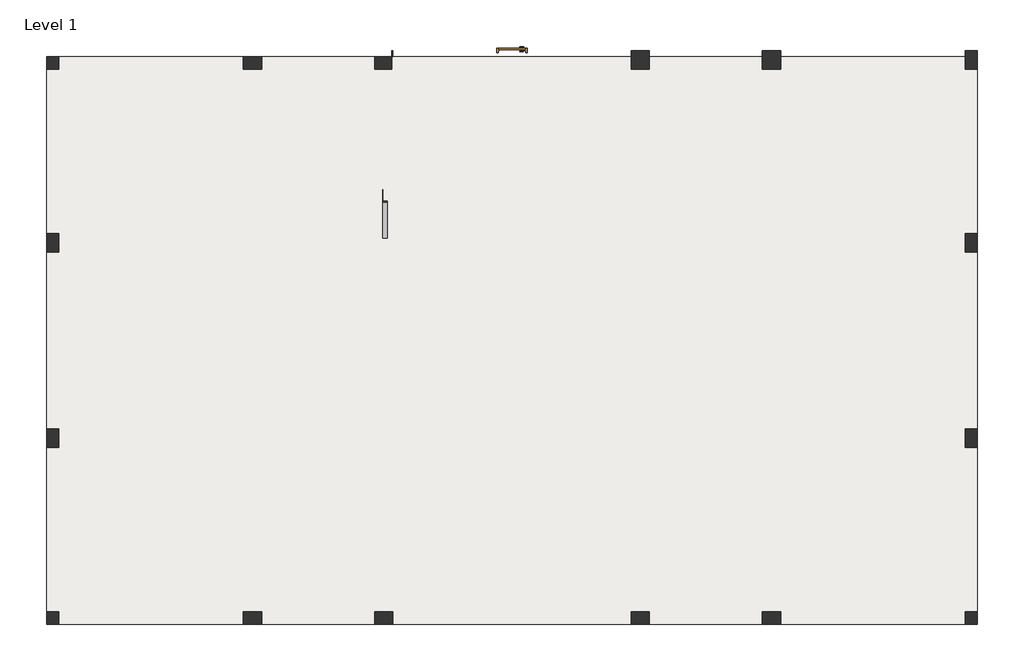
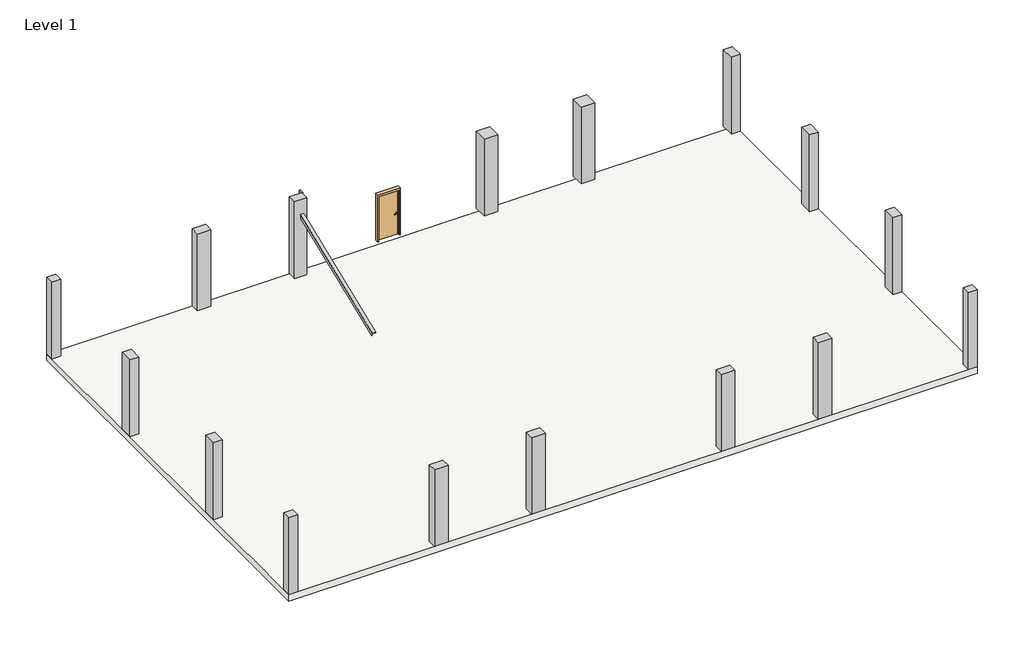
# One storey: 16 columns, 1 door, 1 member, 1 slab.
"""IFC4 building model written with IfcOpenShell, lengths in millimetres."""

import ifcopenshell
import ifcopenshell.guid

model = None  # the IFC model being written
_history = None  # IfcOwnerHistory: only IFC2X3 demands one
_inside = {}  # id of a spatial element -> (the spatial element, [elements in it])
_under = {}  # id of a project, library or spatial element -> (it, [spatial elements below it])
_declared = {}  # id of a project -> (the project, [libraries it declares])
_typed = {}  # id of a type object -> (the type object, [elements of that type])
_made_of = {}  # id of a material, layer set ... -> (it, [elements and type objects made of it])


def new_model(schema):
    """Start an empty IFC model of exactly this schema.

    Asked for "IFC4X3", IfcOpenShell would pick the latest addendum, in which some entities
    have other attributes; the version numbers below select the first issue.
    IFC2X3 requires an IfcOwnerHistory on every rooted entity: one is made here for all.
    """
    global model, _history
    if schema == "IFC4X3":
        model = ifcopenshell.file(schema_version=(4, 3, 0, 0))
    else:
        model = ifcopenshell.file(schema=schema)
    _inside.clear()
    _under.clear()
    _declared.clear()
    _typed.clear()
    _made_of.clear()
    _history = None
    if model.schema == "IFC2X3":
        org = make("IfcOrganization", Name="unknown")
        user = make(
            "IfcPersonAndOrganization",
            ThePerson=make("IfcPerson", FamilyName="unknown"),
            TheOrganization=org,
        )
        app = make(
            "IfcApplication",
            ApplicationDeveloper=org,
            Version="unknown",
            ApplicationFullName="unknown",
            ApplicationIdentifier="unknown",
        )
        _history = make(
            "IfcOwnerHistory",
            OwningUser=user,
            OwningApplication=app,
            ChangeAction="ADDED",
            CreationDate=0,
        )
    return model


def make(cls, **values):
    """One entity of the class cls with the attributes given. An attribute that is None is left unset."""
    return model.create_entity(
        cls, **{name: value for name, value in values.items() if value is not None}
    )


def rooted(cls, **values):
    """An entity with a GlobalId (a new one), such as an element, a storey or a relation."""
    return make(cls, GlobalId=ifcopenshell.guid.new(), OwnerHistory=_history, **values)


def si_unit(unit_type, name, prefix=None):
    """IfcSIUnit, for example si_unit("LENGTHUNIT", "METRE", prefix="MILLI")."""
    return make("IfcSIUnit", UnitType=unit_type, Prefix=prefix, Name=name)


def assignment(units):
    """IfcUnitAssignment: the units of a project."""
    return None if units is None else make("IfcUnitAssignment", Units=units)


def point(xyz):
    """IfcCartesianPoint."""
    return None if xyz is None else make("IfcCartesianPoint", Coordinates=xyz)


def direction(xyz):
    """IfcDirection."""
    return None if xyz is None else make("IfcDirection", DirectionRatios=xyz)


def frame(location, z_axis=None, x_axis=None):
    """IfcAxis2Placement3D, a coordinate frame: its origin and axes. An axis left out is left unset."""
    return make(
        "IfcAxis2Placement3D",
        Location=point(location),
        Axis=direction(z_axis),
        RefDirection=direction(x_axis),
    )


def frame_2d(location, x_axis=None):
    """IfcAxis2Placement2D, a coordinate frame in the plane: its origin and x axis."""
    return make(
        "IfcAxis2Placement2D", Location=point(location), RefDirection=direction(x_axis)
    )


def origin():
    """The frame at (0, 0, 0) with its axes left unset."""
    return frame((0.0, 0.0, 0.0))


def origin_with_axes():
    """The frame at (0, 0, 0) with the z axis (0, 0, 1) and the x axis (1, 0, 0) written out."""
    return frame((0.0, 0.0, 0.0), z_axis=(0.0, 0.0, 1.0), x_axis=(1.0, 0.0, 0.0))


def place(relative_to, where):
    """IfcLocalPlacement: puts the frame where relative to a parent placement (None: the world)."""
    return make(
        "IfcLocalPlacement", PlacementRelTo=relative_to, RelativePlacement=where
    )


def context(
    kind, dimensions, precision=None, world=None, true_north=None, identifier=None
):
    """IfcGeometricRepresentationContext, for example the 3D "Model" context."""
    return make(
        "IfcGeometricRepresentationContext",
        ContextIdentifier=identifier,
        ContextType=kind,
        CoordinateSpaceDimension=dimensions,
        Precision=precision,
        WorldCoordinateSystem=world,
        TrueNorth=true_north,
    )


def project(units=None, contexts=None):
    """IfcProject with its units and contexts."""
    return rooted(
        "IfcProject",
        Name="project",
        RepresentationContexts=contexts,
        UnitsInContext=assignment(units),
    )


def spatial(cls, under=None, at=None, **own):
    """A site, building, storey or space (cls), placed at a placement, below another one or the project."""
    s = rooted(cls, ObjectPlacement=at, **own)
    if under is not None:
        _under.setdefault(under.id(), (under, []))[1].append(s)
    return s


def polyline(points):
    """IfcPolyline through the points."""
    return make("IfcPolyline", Points=[point(p) for p in points])


def circle_curve(where, radius):
    """IfcCircle in the frame where."""
    return make("IfcCircle", Position=where, Radius=radius)


def ellipse_curve(where, semi_axis1, semi_axis2):
    """IfcEllipse in the frame where."""
    return make(
        "IfcEllipse", Position=where, SemiAxis1=semi_axis1, SemiAxis2=semi_axis2
    )


def trimmed(basis, trim1, trim2, sense, master):
    """IfcTrimmedCurve: the piece of a basis curve between two trims."""
    return make(
        "IfcTrimmedCurve",
        BasisCurve=basis,
        Trim1=trim1,
        Trim2=trim2,
        SenseAgreement=sense,
        MasterRepresentation=master,
    )


def segment(curve, same_sense, transition):
    """IfcCompositeCurveSegment."""
    return make(
        "IfcCompositeCurveSegment",
        Transition=transition,
        SameSense=same_sense,
        ParentCurve=curve,
    )


def composite_curve(segments, self_intersect=None):
    """IfcCompositeCurve: segments joined end to end."""
    return make("IfcCompositeCurve", Segments=segments, SelfIntersect=self_intersect)


def outline(outer, holes=None, kind="AREA"):
    """IfcArbitraryClosedProfileDef: a profile drawn as a closed curve; with holes, ...WithVoids."""
    if holes is None:
        return make("IfcArbitraryClosedProfileDef", ProfileType=kind, OuterCurve=outer)
    return make(
        "IfcArbitraryProfileDefWithVoids",
        ProfileType=kind,
        OuterCurve=outer,
        InnerCurves=holes,
    )


def extrude(swept, where, along, depth):
    """IfcExtrudedAreaSolid: the profile swept, set in the frame where, extruded along a direction by depth."""
    return make(
        "IfcExtrudedAreaSolid",
        SweptArea=swept,
        Position=where,
        ExtrudedDirection=direction(along),
        Depth=depth,
    )


def faces_of(points, faces, orient=None, outer=None):
    """IfcFace entities. A face is a list of loops; a loop is a list of indices into points, from 0.

    orient and outer hold one flag for each loop. By default every Orientation is true, the
    first loop of a face is its IfcFaceOuterBound and the others are IfcFaceBound.
    """
    made = []
    for i, loops in enumerate(faces):
        bounds = []
        for j, loop in enumerate(loops):
            is_outer = j == 0 if outer is None else outer[i][j]
            bounds.append(
                make(
                    "IfcFaceOuterBound" if is_outer else "IfcFaceBound",
                    Bound=make("IfcPolyLoop", Polygon=[points[k] for k in loop]),
                    Orientation=True if orient is None else orient[i][j],
                )
            )
        made.append(make("IfcFace", Bounds=bounds))
    return made


def faceted_brep(points, faces, orient=None, outer=None, voids=None):
    """IfcFacetedBrep: a solid bounded by flat faces; with voids (closed shells), ...WithVoids."""
    shared = [point(p) for p in points]
    hull = make("IfcClosedShell", CfsFaces=faces_of(shared, faces, orient, outer))
    if voids is None:
        return make("IfcFacetedBrep", Outer=hull)
    return make(
        "IfcFacetedBrepWithVoids",
        Outer=hull,
        Voids=[
            make(cls, CfsFaces=faces_of(shared, fs, o, b)) for cls, fs, o, b in voids
        ],
    )


def shape(context_of_items, identifier, shape_type, items):
    """IfcShapeRepresentation: the items that make up one representation, for example the "Body"."""
    return make(
        "IfcShapeRepresentation",
        ContextOfItems=context_of_items,
        RepresentationIdentifier=identifier,
        RepresentationType=shape_type,
        Items=items,
    )


def source(mapping_origin, context_of_items, identifier, shape_type, items):
    """IfcRepresentationMap: a shape defined once, which mapped items show again and again."""
    return make(
        "IfcRepresentationMap",
        MappingOrigin=mapping_origin,
        MappedRepresentation=shape(context_of_items, identifier, shape_type, items),
    )


def transform(
    local_origin,
    x_axis=None,
    y_axis=None,
    z_axis=None,
    scale=None,
    scale2=None,
    scale3=None,
    uniform=True,
):
    """IfcCartesianTransformationOperator3D, or its non-uniform kind. x_axis, y_axis, z_axis: its Axis1, 2, 3."""
    if uniform:
        return make(
            "IfcCartesianTransformationOperator3D",
            Axis1=direction(x_axis),
            Axis2=direction(y_axis),
            LocalOrigin=point(local_origin),
            Scale=scale,
            Axis3=direction(z_axis),
        )
    return make(
        "IfcCartesianTransformationOperator3DnonUniform",
        Axis1=direction(x_axis),
        Axis2=direction(y_axis),
        LocalOrigin=point(local_origin),
        Scale=scale,
        Axis3=direction(z_axis),
        Scale2=scale2,
        Scale3=scale3,
    )


def mapped(mapping_source, mapping_target):
    """IfcMappedItem: shows the shape of a source again, moved by a transform."""
    return make(
        "IfcMappedItem", MappingSource=mapping_source, MappingTarget=mapping_target
    )


def made_of(thing, what):
    """Note that an element or type object is made of a material, layer set ...; save() writes the relation."""
    if what is not None:
        _made_of.setdefault(what.id(), (what, []))[1].append(thing)
    return thing


def element(
    cls,
    number,
    at=None,
    inside=None,
    cuts=None,
    type_object=None,
    material=None,
    context=None,
    identifier="Body",
    shape_type=None,
    held_by="IfcProductDefinitionShape",
    body=None,
    shapes=None,
    **own,
):
    """One element of the class cls, such as IfcWall. Its Tag is "e" and its number.

    at: its placement. inside: the storey or other place that contains it. cuts: it is an
    opening in that element (IfcRelVoidsElement). A single representation is given by context,
    identifier, shape_type and body (its items); several are given by shapes. held_by: the class
    of the entity that holds the representations. save() writes the other relations.
    """
    e = rooted(cls, Tag="e%d" % number, ObjectPlacement=at, **own)
    if body is not None:
        shapes = [shape(context, identifier, shape_type, body)]
    if shapes is not None:
        e.Representation = make(held_by, Representations=shapes)
    if inside is not None:
        _inside.setdefault(inside.id(), (inside, []))[1].append(e)
    if cuts is not None:
        rooted(
            "IfcRelVoidsElement", RelatingBuildingElement=cuts, RelatedOpeningElement=e
        )
    if type_object is not None:
        _typed.setdefault(type_object.id(), (type_object, []))[1].append(e)
    return made_of(e, material)


def aggregate(whole, parts):
    """IfcRelAggregates: a whole, such as a stair, and the parts it consists of."""
    return rooted("IfcRelAggregates", RelatingObject=whole, RelatedObjects=parts)


def save(model, path):
    """Write the relations noted so far, then the file.

    IfcRelAggregates (storeys below a building ...), IfcRelContainedInSpatialStructure (elements
    in a storey), IfcRelDefinesByType, IfcRelAssociatesMaterial and IfcRelDeclares: one each for
    every whole, place, type object, material and project.
    """
    for whole, parts in _under.values():
        aggregate(whole, parts)
    for where, things in _inside.values():
        rooted(
            "IfcRelContainedInSpatialStructure",
            RelatedElements=things,
            RelatingStructure=where,
        )
    for kind, things in _typed.values():
        rooted("IfcRelDefinesByType", RelatedObjects=things, RelatingType=kind)
    for what, things in _made_of.values():
        rooted("IfcRelAssociatesMaterial", RelatedObjects=things, RelatingMaterial=what)
    for by, libraries in _declared.values():
        rooted("IfcRelDeclares", RelatingContext=by, RelatedDefinitions=libraries)
    model.write(path)


def plane_surface(at):
    """IfcPlane: the flat surface through the origin of the frame at, square to its z axis."""
    return make("IfcPlane", Position=at)


def cylinder_surface(at, radius):
    """IfcCylindricalSurface: all points at the distance radius from the z axis of the frame at."""
    return make("IfcCylindricalSurface", Position=at, Radius=radius)


def revolved_surface(curve, axis_point, axis_direction):
    """IfcSurfaceOfRevolution: the curve turned about the line through axis_point along axis_direction."""
    return make(
        "IfcSurfaceOfRevolution",
        SweptCurve=make("IfcArbitraryOpenProfileDef", ProfileType="CURVE", Curve=curve),
        AxisPosition=make("IfcAxis1Placement", Location=point(axis_point), Axis=direction(axis_direction)),
    )


def advanced_brep(points, edges, surfaces, faces):
    """IfcAdvancedBrep: a solid bounded by faces that lie on surfaces and meet in shared edges.

    An edge is (start, end): straight between two places in points (the first is 0);
    or (start, end, curve); or (start, end, curve, False) where it runs against its curve.
    A face is (place in surfaces, loops), or (place, loops, False) where it looks against
    its surface's normal. A loop lists edges by number (the first is 1), with a minus sign
    where the edge is run from its end to its start. The first loop is the outer one.
    """
    corners = [point(p) for p in points]
    vertices = [make("IfcVertexPoint", VertexGeometry=c) for c in corners]
    made = []
    for start, end, *more in edges:
        made.append(
            make(
                "IfcEdgeCurve",
                EdgeStart=vertices[start],
                EdgeEnd=vertices[end],
                EdgeGeometry=more[0] if more else make("IfcPolyline", Points=[corners[start], corners[end]]),
                SameSense=more[1] if len(more) > 1 else True,
            )
        )
    hull = []
    for where, loops, *sense in faces:
        bounds = []
        for j, loop in enumerate(loops):
            ring = [make("IfcOrientedEdge", EdgeElement=made[abs(k) - 1], Orientation=k > 0) for k in loop]
            bounds.append(
                make(
                    "IfcFaceOuterBound" if j == 0 else "IfcFaceBound",
                    Bound=make("IfcEdgeLoop", EdgeList=ring),
                    Orientation=True,
                )
            )
        hull.append(make("IfcAdvancedFace", Bounds=bounds, FaceSurface=surfaces[where], SameSense=sense[0] if sense else True))
    return make("IfcAdvancedBrep", Outer=make("IfcClosedShell", CfsFaces=hull))


def door_58febf71(model_context):
    return source(origin(), model_context, "Body", "SolidModel", [
        advanced_brep(
        [(-392.190625, -76.1375, 1016.0), (-372.190625, -76.1375, 1016.0), (-392.190625, -46.1375, 1016.0), (-372.190625, -46.1375, 1016.0), (-367.190625, -41.1375, 1016.0), (-367.190625, -21.1375, 1016.0), (-262.190625, -21.1375, 1016.0), (-262.190625, -41.1375, 1016.0)],
        [
            (0, 1, circle_curve(frame((-382.190625, -76.1375, 1016.0), z_axis=(0.0, -1.0, 0.0), x_axis=(1.0, 0.0, 0.0)), 10.0)),
            (1, 0, circle_curve(frame((-382.190625, -76.1375, 1016.0), z_axis=(0.0, -1.0, 0.0), x_axis=(1.0, 0.0, 0.0)), 10.0)),
            (0, 2),
            (2, 3, circle_curve(frame((-382.190625, -46.1375, 1016.0), z_axis=(0.0, -1.0, 0.0), x_axis=(1.0, 0.0, 0.0)), 10.0)),
            (3, 1),
            (3, 2, circle_curve(frame((-382.190625, -46.1375, 1016.0), z_axis=(0.0, -1.0, 0.0), x_axis=(1.0, 0.0, 0.0)), 10.0)),
            (4, 3, circle_curve(frame((-367.190625, -46.1375, 1016.0), z_axis=(0.0, 0.0, 1.0), x_axis=(-1.0, 0.0, 0.0)), 5.0)),
            (2, 5, circle_curve(frame((-367.190625, -46.1375, 1016.0), z_axis=(0.0, 0.0, -1.0), x_axis=(-1.0, 0.0, 0.0)), 25.0)),
            (5, 4, circle_curve(frame((-367.190625, -31.1375, 1016.0), z_axis=(-1.0, 0.0, 0.0), x_axis=(0.0, -1.0, 0.0)), 10.0)),
            (4, 5, circle_curve(frame((-367.190625, -31.1375, 1016.0), z_axis=(-1.0, 0.0, 0.0), x_axis=(0.0, -1.0, 0.0)), 10.0)),
            (6, 7, circle_curve(frame((-262.190625, -31.1375, 1016.0), z_axis=(1.0, 0.0, 0.0), x_axis=(0.0, -1.0, 0.0)), 10.0)),
            (7, 6, circle_curve(frame((-262.190625, -31.1375, 1016.0), z_axis=(1.0, 0.0, 0.0), x_axis=(0.0, -1.0, 0.0)), 10.0)),
            (5, 6),
            (7, 4),
        ],
        [
            plane_surface(frame((-382.190625, -76.1375, 1016.0), z_axis=(0.0, -1.0, 0.0), x_axis=(0.0, 0.0, 1.0))),
            cylinder_surface(frame((-382.190625, -76.1375, 1016.0), z_axis=(0.0, -1.0, 0.0), x_axis=(1.0, 0.0, 0.0)), 10.0),
            revolved_surface(trimmed(ellipse_curve(frame((-382.190625, -46.1375, 1016.0), z_axis=(0.0, -1.0, 0.0), x_axis=(1.0, 0.0, 0.0)), 10.0, 10.0), [point((-392.190625, -46.1375, 1016.0))], [point((-372.190625, -46.1375, 1016.0))], True, "CARTESIAN"), (-367.190625, -46.1375, 1016.0), (0.0, 0.0, -1.0)),
            revolved_surface(trimmed(ellipse_curve(frame((-382.190625, -46.1375, 1016.0), z_axis=(0.0, -1.0, 0.0), x_axis=(1.0, 0.0, 0.0)), 10.0, 10.0), [point((-372.190625, -46.1375, 1016.0))], [point((-392.190625, -46.1375, 1016.0))], True, "CARTESIAN"), (-367.190625, -46.1375, 1016.0), (0.0, 0.0, -1.0)),
            plane_surface(frame((-262.190625, -31.1375, 1016.0), z_axis=(1.0, 0.0, 0.0), x_axis=(0.0, 0.0, 1.0))),
            cylinder_surface(frame((-367.190625, -31.1375, 1016.0), z_axis=(-1.0, 0.0, 0.0), x_axis=(0.0, -1.0, 0.0)), 10.0),
        ],
        [
            (0, [[1, 2]]),
            (1, [[-1, 3, 4, 5]]),
            (1, [[-2, -5, 6, -3]]),
            (2, [[7, -4, 8, 9]]),
            (3, [[-8, -6, -7, 10]]),
            (4, [[11, 12]]),
            (5, [[-9, 13, -12, 14]]),
            (5, [[-10, -14, -11, -13]]),
        ],
    ),
        extrude(outline(composite_curve([segment(trimmed(circle_curve(frame_2d((1016.0, -384.690625)), 30.0), [point((1016.0, -414.690625))], [point((1016.0, -354.690625))], False, "CARTESIAN"), True, "CONTINUOUS"), segment(trimmed(circle_curve(frame_2d((1016.0, -384.690625)), 30.0), [point((1016.0, -354.690625))], [point((1016.0, -414.690625))], False, "CARTESIAN"), True, "CONTINUOUS")], self_intersect=False)), frame((0.0, -84.1375, 0.0), z_axis=(0.0, 1.0, 0.0), x_axis=(0.0, 0.0, 1.0)), (0.0, 0.0, 1.0), 8.0),
        advanced_brep(
        [(-392.190625, -136.5875, 1016.0), (-372.190625, -136.5875, 1016.0), (-372.190625, -166.5875, 1016.0), (-392.190625, -166.5875, 1016.0), (-367.190625, -171.5875, 1016.0), (-367.190625, -191.5875, 1016.0), (-262.190625, -191.5875, 1016.0), (-262.190625, -171.5875, 1016.0)],
        [
            (0, 1, circle_curve(frame((-382.190625, -136.5875, 1016.0), z_axis=(0.0, 1.0, 0.0), x_axis=(1.0, 0.0, 0.0)), 10.0)),
            (1, 0, circle_curve(frame((-382.190625, -136.5875, 1016.0), z_axis=(0.0, 1.0, 0.0), x_axis=(1.0, 0.0, 0.0)), 10.0)),
            (1, 2),
            (2, 3, circle_curve(frame((-382.190625, -166.5875, 1016.0), z_axis=(0.0, 1.0, 0.0), x_axis=(1.0, 0.0, 0.0)), 10.0)),
            (3, 0),
            (3, 2, circle_curve(frame((-382.190625, -166.5875, 1016.0), z_axis=(0.0, 1.0, 0.0), x_axis=(1.0, 0.0, 0.0)), 10.0)),
            (4, 5, circle_curve(frame((-367.190625, -181.5875, 1016.0), z_axis=(-1.0, 0.0, 0.0), x_axis=(0.0, 1.0, 0.0)), 10.0)),
            (5, 3, circle_curve(frame((-367.190625, -166.5875, 1016.0), z_axis=(0.0, 0.0, -1.0), x_axis=(-1.0, 0.0, 0.0)), 25.0)),
            (2, 4, circle_curve(frame((-367.190625, -166.5875, 1016.0), z_axis=(0.0, 0.0, 1.0), x_axis=(-1.0, 0.0, 0.0)), 5.0)),
            (5, 4, circle_curve(frame((-367.190625, -181.5875, 1016.0), z_axis=(-1.0, 0.0, 0.0), x_axis=(0.0, 1.0, 0.0)), 10.0)),
            (6, 7, circle_curve(frame((-262.190625, -181.5875, 1016.0), z_axis=(1.0, 0.0, 0.0), x_axis=(0.0, 1.0, 0.0)), 10.0)),
            (7, 6, circle_curve(frame((-262.190625, -181.5875, 1016.0), z_axis=(1.0, 0.0, 0.0), x_axis=(0.0, 1.0, 0.0)), 10.0)),
            (4, 7),
            (6, 5),
        ],
        [
            plane_surface(frame((-382.190625, -136.5875, 1016.0), z_axis=(0.0, 1.0, 0.0), x_axis=(0.0, 0.0, 1.0))),
            cylinder_surface(frame((-382.190625, -136.5875, 1016.0), z_axis=(0.0, 1.0, 0.0), x_axis=(1.0, 0.0, 0.0)), 10.0),
            revolved_surface(trimmed(ellipse_curve(frame((-382.190625, -166.5875, 1016.0), z_axis=(0.0, -1.0, 0.0), x_axis=(1.0, 0.0, 0.0)), 10.0, 10.0), [point((-392.190625, -166.5875, 1016.0))], [point((-372.190625, -166.5875, 1016.0))], True, "CARTESIAN"), (-367.190625, -166.5875, 1016.0), (0.0, 0.0, -1.0)),
            revolved_surface(trimmed(ellipse_curve(frame((-382.190625, -166.5875, 1016.0), z_axis=(0.0, -1.0, 0.0), x_axis=(1.0, 0.0, 0.0)), 10.0, 10.0), [point((-372.190625, -166.5875, 1016.0))], [point((-392.190625, -166.5875, 1016.0))], True, "CARTESIAN"), (-367.190625, -166.5875, 1016.0), (0.0, 0.0, -1.0)),
            plane_surface(frame((-262.190625, -181.5875, 1016.0), z_axis=(1.0, 0.0, 0.0), x_axis=(0.0, 0.0, 1.0))),
            cylinder_surface(frame((-367.190625, -181.5875, 1016.0), z_axis=(-1.0, 0.0, 0.0), x_axis=(0.0, 1.0, 0.0)), 10.0),
        ],
        [
            (0, [[1, 2]]),
            (1, [[3, 4, 5, -2]]),
            (1, [[-5, 6, -3, -1]]),
            (2, [[7, 8, -4, 9]]),
            (3, [[10, -9, -6, -8]]),
            (4, [[11, 12]]),
            (5, [[13, -11, 14, -7]]),
            (5, [[-14, -12, -13, -10]]),
        ],
    ),
        extrude(outline(composite_curve([segment(trimmed(circle_curve(frame_2d((1016.0, -384.690625)), 30.0), [point((1016.0, -414.690625))], [point((1016.0, -354.690625))], False, "CARTESIAN"), True, "CONTINUOUS"), segment(trimmed(circle_curve(frame_2d((1016.0, -384.690625)), 30.0), [point((1016.0, -354.690625))], [point((1016.0, -414.690625))], False, "CARTESIAN"), True, "CONTINUOUS")], self_intersect=False)), frame((0.0, -136.5875, 0.0), z_axis=(0.0, 1.0, 0.0), x_axis=(0.0, 0.0, 1.0)), (0.0, 0.0, 1.0), 8.0),
        faceted_brep([(457.2, -79.375, 0.0), (441.325, -79.375, 0.0), (441.325, -31.75, 0.0), (457.2, -31.75, 0.0), (457.2, 17.4625, 0.0), (508.0, 17.4625, 0.0), (508.0, -128.5875, 0.0), (457.2, -128.5875, 0.0), (457.2, -128.5875, 2133.6), (457.2, -79.375, 2133.6), (508.0, -128.5875, 2235.2), (-508.0, -128.5875, 2235.2), (-508.0, -128.5875, 0.0), (-457.2, -128.5875, 0.0), (-457.2, -128.5875, 2133.6), (508.0, 17.4625, 2235.2), (457.2, 17.4625, 2133.6), (-457.2, 17.4625, 2133.6), (-457.2, 17.4625, 0.0), (-508.0, 17.4625, 0.0), (-508.0, 17.4625, 2235.2), (457.2, -31.75, 2133.6), (441.325, -31.75, 2117.725), (-441.325, -31.75, 2117.725), (-441.325, -31.75, 0.0), (-457.2, -31.75, 0.0), (-457.2, -31.75, 2133.6), (441.325, -79.375, 2117.725), (-457.2, -79.375, 2133.6), (-457.2, -79.375, 0.0), (-441.325, -79.375, 0.0), (-441.325, -79.375, 2117.725)], [[[0, 1, 2, 3, 4, 5, 6, 7]], [[7, 8, 9, 0]], [[6, 10, 11, 12, 13, 14, 8, 7]], [[5, 15, 10, 6]], [[4, 16, 17, 18, 19, 20, 15, 5]], [[3, 21, 16, 4]], [[2, 22, 23, 24, 25, 26, 21, 3]], [[1, 27, 22, 2]], [[0, 9, 28, 29, 30, 31, 27, 1]], [[8, 14, 28, 9]], [[16, 21, 26, 17]], [[22, 27, 31, 23]], [[12, 19, 18, 25, 24, 30, 29, 13]], [[13, 29, 28, 14]], [[11, 20, 19, 12]], [[17, 26, 25, 18]], [[23, 31, 30, 24]], [[15, 20, 11, 10]]]),
        extrude(outline(polyline([(457.2, -84.1375), (457.2, -128.5875), (-457.2, -128.5875), (-457.2, -84.1375), (457.2, -84.1375)])), origin_with_axes(), (0.0, 0.0, 1.0), 2133.6),
    ])


def l_angle_l6x6x3_8_2b984bf3(model_context):
    return source(origin(), model_context, "Body", "SweptSolid", [
        extrude(outline(composite_curve([segment(polyline([(41.148, 41.148), (41.148, -111.252)]), True, "CONTINUOUS"), segment(trimmed(circle_curve(frame_2d((41.148, -101.727)), 9.525), [point((41.148, -111.252))], [point((31.623, -101.727))], False, "CARTESIAN"), True, "CONTINUOUS"), segment(polyline([(31.623, -101.727), (31.623, 22.098)]), True, "CONTINUOUS"), segment(trimmed(circle_curve(frame_2d((22.098, 22.098)), 9.525), [point((31.623, 22.098))], [point((22.098, 31.623))], True, "CARTESIAN"), True, "CONTINUOUS"), segment(polyline([(22.098, 31.623), (-101.727, 31.623)]), True, "CONTINUOUS"), segment(trimmed(circle_curve(frame_2d((-101.727, 41.148)), 9.525), [point((-101.727, 31.623))], [point((-111.252, 41.148))], False, "CARTESIAN"), True, "CONTINUOUS"), segment(polyline([(-111.252, 41.148), (41.148, 41.148)]), True, "CONTINUOUS")], self_intersect=False)), frame((-3088.1296112, 0.0, 0.0), z_axis=(1.0, 0.0, 0.0), x_axis=(0.0, 1.0, 0.0)), (0.0, 0.0, 1.0), 6142.746295),
    ])


model = new_model("IFC4")

# Units and contexts
model_context = context("Model", 3, world=origin())
ifc_project = project(units=[si_unit("LENGTHUNIT", "METRE", prefix="MILLI")], contexts=[model_context])

# Site, building, storey
site = spatial("IfcSite", under=ifc_project)
building = spatial("IfcBuilding", under=site)
storey = spatial("IfcBuildingStorey", under=building, Name="Level 1", Elevation=0.0)

# Columns
placement = place(None, origin())
element("IfcColumn", 1, ObjectType="Rectangular Column : 24\" x 24\"", at=placement, inside=storey, context=model_context, shape_type="SweptSolid", body=[
    extrude(outline(polyline([(-16253.4122732, 9291.5015304), (-16253.4122732, 8885.1015304), (-16659.8122732, 8885.1015304), (-16659.8122732, 9291.5015304), (-16253.4122732, 9291.5015304)])), origin_with_axes(), (0.0, 0.0, 1.0), 3657.6),
])
element("IfcColumn", 2, ObjectType="Rectangular Column : 24\" x 24\"", at=placement, inside=storey, context=model_context, shape_type="SweptSolid", body=[
    extrude(outline(polyline([(-16253.4122732, 3398.7015304), (-16253.4122732, 2789.1015304), (-16659.8122732, 2789.1015304), (-16659.8122732, 3398.7015304), (-16253.4122732, 3398.7015304)])), origin_with_axes(), (0.0, 0.0, 1.0), 3657.6),
])
element("IfcColumn", 3, ObjectType="Rectangular Column : 24\" x 24\"", at=placement, inside=storey, context=model_context, shape_type="SweptSolid", body=[
    extrude(outline(polyline([(-9497.0122732, 8885.1015304), (-10106.6122732, 8885.1015304), (-10106.6122732, 9291.5015304), (-9497.0122732, 9291.5015304), (-9497.0122732, 8885.1015304)])), origin_with_axes(), (0.0, 0.0, 1.0), 3657.6),
])
element("IfcColumn", 4, ObjectType="Rectangular Column : 24\" x 24\"", at=placement, inside=storey, context=model_context, shape_type="SweptSolid", body=[
    extrude(outline(polyline([(-5174.2497732, 9494.7015304), (-5128.2122732, 9494.7015304), (-5128.2122732, 9301.0265304), (-5174.2497732, 9301.0265304), (-5174.2497732, 9494.7015304)])), origin_with_axes(), (0.0, 0.0, 1.0), 3657.6),
    extrude(outline(polyline([(-5737.8122732, 8885.1015304), (-5737.8122732, 9291.5015304), (-5174.2497732, 9291.5015304), (-5174.2497732, 8885.1015304), (-5737.8122732, 8885.1015304)])), origin_with_axes(), (0.0, 0.0, 1.0), 3657.6),
])
element("IfcColumn", 5, ObjectType="Rectangular Column : 24\" x 24\"", at=placement, inside=storey, context=model_context, shape_type="SweptSolid", body=[
    extrude(outline(polyline([(3406.1877268, 9494.7015304), (3406.1877268, 8885.1015304), (2796.5877268, 8885.1015304), (2796.5877268, 9494.7015304), (3406.1877268, 9494.7015304)])), origin_with_axes(), (0.0, 0.0, 1.0), 3657.6),
])
element("IfcColumn", 6, ObjectType="Rectangular Column : 24\" x 24\"", at=placement, inside=storey, context=model_context, shape_type="SweptSolid", body=[
    extrude(outline(polyline([(7774.9877268, 9494.7015304), (7774.9877268, 8885.1015304), (7165.3877268, 8885.1015304), (7165.3877268, 9494.7015304), (7774.9877268, 9494.7015304)])), origin_with_axes(), (0.0, 0.0, 1.0), 3657.6),
])
element("IfcColumn", 7, ObjectType="Rectangular Column : 24\" x 24\"", at=placement, inside=storey, context=model_context, shape_type="SweptSolid", body=[
    extrude(outline(polyline([(13921.7877268, 8885.1015304), (13921.7877268, 9494.7015304), (14328.1877268, 9494.7015304), (14328.1877268, 8885.1015304), (13921.7877268, 8885.1015304)])), origin_with_axes(), (0.0, 0.0, 1.0), 3657.6),
])
element("IfcColumn", 8, ObjectType="Rectangular Column : 24\" x 24\"", at=placement, inside=storey, context=model_context, shape_type="SweptSolid", body=[
    extrude(outline(polyline([(13921.7877268, 2789.1015304), (13921.7877268, 3398.7015304), (14328.1877268, 3398.7015304), (14328.1877268, 2789.1015304), (13921.7877268, 2789.1015304)])), origin_with_axes(), (0.0, 0.0, 1.0), 3657.6),
])
element("IfcColumn", 9, ObjectType="Rectangular Column : 24\" x 24\"", at=placement, inside=storey, context=model_context, shape_type="SweptSolid", body=[
    extrude(outline(polyline([(13921.7877268, -3713.2984696), (13921.7877268, -3103.6984696), (14328.1877268, -3103.6984696), (14328.1877268, -3713.2984696), (13921.7877268, -3713.2984696)])), origin_with_axes(), (0.0, 0.0, 1.0), 3657.6),
])
element("IfcColumn", 10, ObjectType="Rectangular Column : 24\" x 24\"", at=placement, inside=storey, context=model_context, shape_type="SweptSolid", body=[
    extrude(outline(polyline([(13921.7877268, -9606.0984696), (13921.7877268, -9199.6984696), (14328.1877268, -9199.6984696), (14328.1877268, -9606.0984696), (13921.7877268, -9606.0984696)])), origin_with_axes(), (0.0, 0.0, 1.0), 3657.6),
])
element("IfcColumn", 11, ObjectType="Rectangular Column : 24\" x 24\"", at=placement, inside=storey, context=model_context, shape_type="SweptSolid", body=[
    extrude(outline(polyline([(7165.3877268, -9199.6984696), (7774.9877268, -9199.6984696), (7774.9877268, -9606.0984696), (7165.3877268, -9606.0984696), (7165.3877268, -9199.6984696)])), origin_with_axes(), (0.0, 0.0, 1.0), 3657.6),
])
element("IfcColumn", 12, ObjectType="Rectangular Column : 24\" x 24\"", at=placement, inside=storey, context=model_context, shape_type="SweptSolid", body=[
    extrude(outline(polyline([(2796.5877268, -9199.6984696), (3406.1877268, -9199.6984696), (3406.1877268, -9606.0984696), (2796.5877268, -9606.0984696), (2796.5877268, -9199.6984696)])), origin_with_axes(), (0.0, 0.0, 1.0), 3657.6),
])
element("IfcColumn", 13, ObjectType="Rectangular Column : 24\" x 24\"", at=placement, inside=storey, context=model_context, shape_type="SweptSolid", body=[
    extrude(outline(polyline([(-5737.8122732, -9199.6984696), (-5128.2122732, -9199.6984696), (-5128.2122732, -9606.0984696), (-5737.8122732, -9606.0984696), (-5737.8122732, -9199.6984696)])), origin_with_axes(), (0.0, 0.0, 1.0), 3657.6),
])
element("IfcColumn", 14, ObjectType="Rectangular Column : 24\" x 24\"", at=placement, inside=storey, context=model_context, shape_type="SweptSolid", body=[
    extrude(outline(polyline([(-10106.6122732, -9199.6984696), (-9497.0122732, -9199.6984696), (-9497.0122732, -9606.0984696), (-10106.6122732, -9606.0984696), (-10106.6122732, -9199.6984696)])), origin_with_axes(), (0.0, 0.0, 1.0), 3657.6),
])
element("IfcColumn", 15, ObjectType="Rectangular Column : 24\" x 24\"", at=placement, inside=storey, context=model_context, shape_type="SweptSolid", body=[
    extrude(outline(polyline([(-16659.8122732, -9199.6984696), (-16253.4122732, -9199.6984696), (-16253.4122732, -9606.0984696), (-16659.8122732, -9606.0984696), (-16659.8122732, -9199.6984696)])), origin_with_axes(), (0.0, 0.0, 1.0), 3657.6),
])
element("IfcColumn", 16, ObjectType="Rectangular Column : 24\" x 24\"", at=placement, inside=storey, context=model_context, shape_type="SweptSolid", body=[
    extrude(outline(polyline([(-16253.4122732, -3103.6984696), (-16253.4122732, -3713.2984696), (-16659.8122732, -3713.2984696), (-16659.8122732, -3103.6984696), (-16253.4122732, -3103.6984696)])), origin_with_axes(), (0.0, 0.0, 1.0), 3657.6),
])

# Door
door_shape = door_58febf71(model_context)
element("IfcDoor", 17, ObjectType="Door-Passage-Single-Flush : 36\" x 84\"", at=placement, inside=storey, context=model_context, shape_type="MappedRepresentation", body=[
    mapped(door_shape, transform((-1165.8122732, 9442.3140304, 0.0), x_axis=(-1.0, 0.0, 0.0), y_axis=(0.0, -1.0, 0.0), z_axis=(0.0, 0.0, 1.0))),
])

# Member
l_angle_l6x6x3_8_shape = l_angle_l6x6x3_8_2b984bf3(model_context)
element("IfcMember", 18, ObjectType="L-Angle : L6X6X3/8", at=placement, inside=storey, context=model_context, shape_type="MappedRepresentation", body=[
    mapped(l_angle_l6x6x3_8_shape, transform((-5433.0122732, 6141.9015304, 1828.8), x_axis=(0.0, 0.9284766908852565, 0.3713906763541112), y_axis=(-1.0000000000000002, 0.0, 0.0), z_axis=(0.0, -0.3713906763541112, 0.9284766908852565))),
])

# Slab
element("IfcSlab", 19, ObjectType="Generic - 12\"", at=placement, inside=storey, context=model_context, shape_type="SweptSolid", body=[
    extrude(outline(polyline([(-16659.8122732, 9291.5015304), (14328.1877268, 9291.5015304), (14328.1877268, -9606.0984696), (-16659.8122732, -9606.0984696), (-16659.8122732, 9291.5015304)])), frame((0.0, 0.0, -304.8), z_axis=(0.0, 0.0, 1.0), x_axis=(1.0, 0.0, 0.0)), (0.0, 0.0, 1.0), 304.8),
])

save(model, "model.ifc")

# Revit data of these elements
# Type "Rectangular Column : 24\" x 24\""
#   Assembly Code = "B1010200"
#   Depth = 2' - 0"
#   Offset Base = 0' - 0"
#   Offset Top = 0' - 0"
#   Width = 2' - 0"
#   Material = none
# Type "Door-Passage-Single-Flush : 36\" x 84\""
#   Type Mark = "1"
#   Assembly Code = "B2030200"
#   Analytic Construction = "Wooden"
#   Thickness = 0' - 1 3/4"
#   Thermal Resistance (R) = 2.5876 (h·ft²·°F)/BTU
#   Swing Angle [instance default] = 90.00°
#   Strike Height = 3' - 4"
#   Rough Width [instance default] = 3' - 4"
#   Rough Height [instance default] = 7' - 4"
#   MF Opening Height [instance default] = 0' - 4"
#   MF Opening Width [instance default] = 0' - 4"
#   Inset Calculate [instance default] = 0' - 4"
#   Masonry Inset [instance default] = 0' - 1"
#   Height = 7' - 0"
#   Width = 3' - 0"
#   Heat Transfer Coefficient (U) = 0.3865 BTU/(h·ft²·°F)
#   Masonry Frame Depth = 0' - 5 3/4"
#   Define Thermal Properties by = 1
#   Masonry Frame [instance default] = yes
#   Function = 1
#   Dry Wall Frame [instance default] = no
#   Panel Material = Wood - Birch
#   Frame Material = Metal - Paint Finish - Grey
#   Door Handle Material = Aluminum
#   Visual Light Transmittance = 0
#   Solar Heat Gain Coefficient = 0
#   Wall Closure = (empty or 0)
# Type "L-Angle : L6X6X3/8"
#   Assembly Code = "B10"
#   k = 0' - 0 7/8"
#   W = 14.9
#   Length [instance default] = 5' - 0"
#   b = 0' - 6"
#   d = 0' - 6"
#   t = 0' - 0 3/8"
#   x = 0' - 1.62"
#   y = 0' - 1.62"
#   A = 0.0304167 SF
#   Structural Material [instance default] = Steel ASTM A36
# Type "Generic - 12\""
#   Assembly Code = "B1010"
#   Function = 0
#   Layers, outside or top first: 1' - 0" no material (function 1)
# Elements 1, 2, 3, 4, 7, 8, 9, 10, 11, 12, 13, 14, 15, 16 (IfcColumn, "Rectangular Column : 24\" x 24\"")
#   Phase Created = New Construction
#   Materials on its faces: "Default Wall"
# Elements 5, 6 (IfcColumn, "Rectangular Column : 24\" x 24\"")
#   Phase Created = New Construction
# Element 17 (IfcDoor, "Door-Passage-Single-Flush : 36\" x 84\"")
#   Swing Angle = 90.00°
#   Rough Width = 3' - 4"
#   Rough Height = 7' - 4"
#   Masonry Inset = 0' - 1"
#   MF Opening Width = 0' - 4"
#   MF Opening Height = 0' - 4"
#   Inset Calculate = 0' - 4"
#   Masonry Frame = yes
#   Dry Wall Frame = no
#   Phase Created = New Construction
#   Materials on its faces: "Aluminum", "Metal - Paint Finish - Grey", "Wood - Birch"
# Element 18 (IfcMember, "L-Angle : L6X6X3/8")
#   Structural Material = Steel ASTM A36
#   Phase Created = New Construction
#   Materials on its faces: "Steel ASTM A36"
# Element 19 (IfcSlab, "Generic - 12\"")
#   built-in parameter 1001955 = 1.5708 (stored number, unit not read)
#   Height Offset From Level = 0' - 0"
#   Phase Created = New Construction
#   Materials on its faces: "Default Floor"
# Materials
#   "Wood - Birch": class "Wood", colour RGB 166 116 52, transparency 0, Cost = 0
#   "Metal - Paint Finish - Grey": class "Paint", colour RGB 104 104 104, transparency 0, Cost = 0
#   "Aluminum": class "Metal", colour RGB 247 247 247, transparency 0, Description = "Aluminum 6061", Cost = 0
#   "Steel ASTM A36": class "Metal", colour RGB 199 199 199, transparency 0, Description = "Structural steel, ASTM A36 Grade B, mill finish", Cost = 0
#   "Default Wall": class "Miscellaneous", colour RGB 128 128 128, transparency 0, Cost = 0
#   "Default Floor": class "Miscellaneous", colour RGB 128 128 128, transparency 0, Cost = 0
